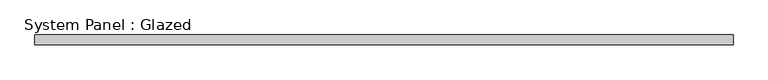
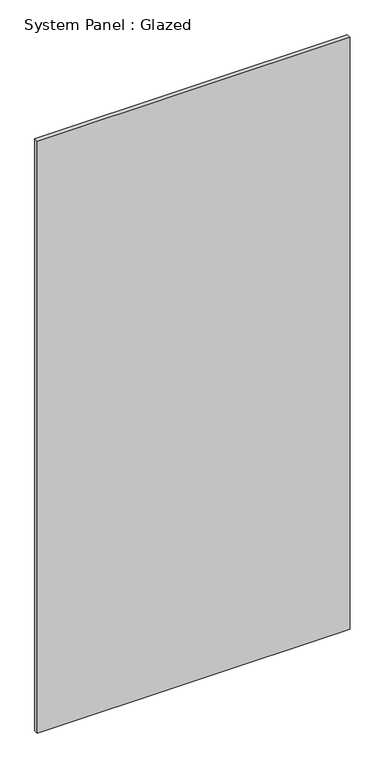
"""IFC4 building model written with IfcOpenShell, lengths in millimetres: plate geometry, System Panel : Glazed."""

import ifcopenshell
import ifcopenshell.guid

model = None  # the IFC model being written
_history = None  # IfcOwnerHistory: only IFC2X3 demands one
_inside = {}  # id of a spatial element -> (the spatial element, [elements in it])
_under = {}  # id of a project, library or spatial element -> (it, [spatial elements below it])
_declared = {}  # id of a project -> (the project, [libraries it declares])
_typed = {}  # id of a type object -> (the type object, [elements of that type])
_made_of = {}  # id of a material, layer set ... -> (it, [elements and type objects made of it])


def new_model(schema):
    """Start an empty IFC model of exactly this schema.

    Asked for "IFC4X3", IfcOpenShell would pick the latest addendum, in which some entities
    have other attributes; the version numbers below select the first issue.
    IFC2X3 requires an IfcOwnerHistory on every rooted entity: one is made here for all.
    """
    global model, _history
    if schema == "IFC4X3":
        model = ifcopenshell.file(schema_version=(4, 3, 0, 0))
    else:
        model = ifcopenshell.file(schema=schema)
    _inside.clear()
    _under.clear()
    _declared.clear()
    _typed.clear()
    _made_of.clear()
    _history = None
    if model.schema == "IFC2X3":
        org = make("IfcOrganization", Name="unknown")
        user = make(
            "IfcPersonAndOrganization",
            ThePerson=make("IfcPerson", FamilyName="unknown"),
            TheOrganization=org,
        )
        app = make(
            "IfcApplication",
            ApplicationDeveloper=org,
            Version="unknown",
            ApplicationFullName="unknown",
            ApplicationIdentifier="unknown",
        )
        _history = make(
            "IfcOwnerHistory",
            OwningUser=user,
            OwningApplication=app,
            ChangeAction="ADDED",
            CreationDate=0,
        )
    return model


def make(cls, **values):
    """One entity of the class cls with the attributes given. An attribute that is None is left unset."""
    return model.create_entity(
        cls, **{name: value for name, value in values.items() if value is not None}
    )


def rooted(cls, **values):
    """An entity with a GlobalId (a new one), such as an element, a storey or a relation."""
    return make(cls, GlobalId=ifcopenshell.guid.new(), OwnerHistory=_history, **values)


def si_unit(unit_type, name, prefix=None):
    """IfcSIUnit, for example si_unit("LENGTHUNIT", "METRE", prefix="MILLI")."""
    return make("IfcSIUnit", UnitType=unit_type, Prefix=prefix, Name=name)


def assignment(units):
    """IfcUnitAssignment: the units of a project."""
    return None if units is None else make("IfcUnitAssignment", Units=units)


def point(xyz):
    """IfcCartesianPoint."""
    return None if xyz is None else make("IfcCartesianPoint", Coordinates=xyz)


def direction(xyz):
    """IfcDirection."""
    return None if xyz is None else make("IfcDirection", DirectionRatios=xyz)


def frame(location, z_axis=None, x_axis=None):
    """IfcAxis2Placement3D, a coordinate frame: its origin and axes. An axis left out is left unset."""
    return make(
        "IfcAxis2Placement3D",
        Location=point(location),
        Axis=direction(z_axis),
        RefDirection=direction(x_axis),
    )


def origin():
    """The frame at (0, 0, 0) with its axes left unset."""
    return frame((0.0, 0.0, 0.0))


def origin_with_axes():
    """The frame at (0, 0, 0) with the z axis (0, 0, 1) and the x axis (1, 0, 0) written out."""
    return frame((0.0, 0.0, 0.0), z_axis=(0.0, 0.0, 1.0), x_axis=(1.0, 0.0, 0.0))


def place(relative_to, where):
    """IfcLocalPlacement: puts the frame where relative to a parent placement (None: the world)."""
    return make(
        "IfcLocalPlacement", PlacementRelTo=relative_to, RelativePlacement=where
    )


def context(
    kind, dimensions, precision=None, world=None, true_north=None, identifier=None
):
    """IfcGeometricRepresentationContext, for example the 3D "Model" context."""
    return make(
        "IfcGeometricRepresentationContext",
        ContextIdentifier=identifier,
        ContextType=kind,
        CoordinateSpaceDimension=dimensions,
        Precision=precision,
        WorldCoordinateSystem=world,
        TrueNorth=true_north,
    )


def project(units=None, contexts=None):
    """IfcProject with its units and contexts."""
    return rooted(
        "IfcProject",
        Name="project",
        RepresentationContexts=contexts,
        UnitsInContext=assignment(units),
    )


def spatial(cls, under=None, at=None, **own):
    """A site, building, storey or space (cls), placed at a placement, below another one or the project."""
    s = rooted(cls, ObjectPlacement=at, **own)
    if under is not None:
        _under.setdefault(under.id(), (under, []))[1].append(s)
    return s


def polyline(points):
    """IfcPolyline through the points."""
    return make("IfcPolyline", Points=[point(p) for p in points])


def outline(outer, holes=None, kind="AREA"):
    """IfcArbitraryClosedProfileDef: a profile drawn as a closed curve; with holes, ...WithVoids."""
    if holes is None:
        return make("IfcArbitraryClosedProfileDef", ProfileType=kind, OuterCurve=outer)
    return make(
        "IfcArbitraryProfileDefWithVoids",
        ProfileType=kind,
        OuterCurve=outer,
        InnerCurves=holes,
    )


def extrude(swept, where, along, depth):
    """IfcExtrudedAreaSolid: the profile swept, set in the frame where, extruded along a direction by depth."""
    return make(
        "IfcExtrudedAreaSolid",
        SweptArea=swept,
        Position=where,
        ExtrudedDirection=direction(along),
        Depth=depth,
    )


def shape(context_of_items, identifier, shape_type, items):
    """IfcShapeRepresentation: the items that make up one representation, for example the "Body"."""
    return make(
        "IfcShapeRepresentation",
        ContextOfItems=context_of_items,
        RepresentationIdentifier=identifier,
        RepresentationType=shape_type,
        Items=items,
    )


def source(mapping_origin, context_of_items, identifier, shape_type, items):
    """IfcRepresentationMap: a shape defined once, which mapped items show again and again."""
    return make(
        "IfcRepresentationMap",
        MappingOrigin=mapping_origin,
        MappedRepresentation=shape(context_of_items, identifier, shape_type, items),
    )


def transform(
    local_origin,
    x_axis=None,
    y_axis=None,
    z_axis=None,
    scale=None,
    scale2=None,
    scale3=None,
    uniform=True,
):
    """IfcCartesianTransformationOperator3D, or its non-uniform kind. x_axis, y_axis, z_axis: its Axis1, 2, 3."""
    if uniform:
        return make(
            "IfcCartesianTransformationOperator3D",
            Axis1=direction(x_axis),
            Axis2=direction(y_axis),
            LocalOrigin=point(local_origin),
            Scale=scale,
            Axis3=direction(z_axis),
        )
    return make(
        "IfcCartesianTransformationOperator3DnonUniform",
        Axis1=direction(x_axis),
        Axis2=direction(y_axis),
        LocalOrigin=point(local_origin),
        Scale=scale,
        Axis3=direction(z_axis),
        Scale2=scale2,
        Scale3=scale3,
    )


def mapped(mapping_source, mapping_target):
    """IfcMappedItem: shows the shape of a source again, moved by a transform."""
    return make(
        "IfcMappedItem", MappingSource=mapping_source, MappingTarget=mapping_target
    )


def made_of(thing, what):
    """Note that an element or type object is made of a material, layer set ...; save() writes the relation."""
    if what is not None:
        _made_of.setdefault(what.id(), (what, []))[1].append(thing)
    return thing


def element(
    cls,
    number,
    at=None,
    inside=None,
    cuts=None,
    type_object=None,
    material=None,
    context=None,
    identifier="Body",
    shape_type=None,
    held_by="IfcProductDefinitionShape",
    body=None,
    shapes=None,
    **own,
):
    """One element of the class cls, such as IfcWall. Its Tag is "e" and its number.

    at: its placement. inside: the storey or other place that contains it. cuts: it is an
    opening in that element (IfcRelVoidsElement). A single representation is given by context,
    identifier, shape_type and body (its items); several are given by shapes. held_by: the class
    of the entity that holds the representations. save() writes the other relations.
    """
    e = rooted(cls, Tag="e%d" % number, ObjectPlacement=at, **own)
    if body is not None:
        shapes = [shape(context, identifier, shape_type, body)]
    if shapes is not None:
        e.Representation = make(held_by, Representations=shapes)
    if inside is not None:
        _inside.setdefault(inside.id(), (inside, []))[1].append(e)
    if cuts is not None:
        rooted(
            "IfcRelVoidsElement", RelatingBuildingElement=cuts, RelatedOpeningElement=e
        )
    if type_object is not None:
        _typed.setdefault(type_object.id(), (type_object, []))[1].append(e)
    return made_of(e, material)


def aggregate(whole, parts):
    """IfcRelAggregates: a whole, such as a stair, and the parts it consists of."""
    return rooted("IfcRelAggregates", RelatingObject=whole, RelatedObjects=parts)


def save(model, path):
    """Write the relations noted so far, then the file.

    IfcRelAggregates (storeys below a building ...), IfcRelContainedInSpatialStructure (elements
    in a storey), IfcRelDefinesByType, IfcRelAssociatesMaterial and IfcRelDeclares: one each for
    every whole, place, type object, material and project.
    """
    for whole, parts in _under.values():
        aggregate(whole, parts)
    for where, things in _inside.values():
        rooted(
            "IfcRelContainedInSpatialStructure",
            RelatedElements=things,
            RelatingStructure=where,
        )
    for kind, things in _typed.values():
        rooted("IfcRelDefinesByType", RelatedObjects=things, RelatingType=kind)
    for what, things in _made_of.values():
        rooted("IfcRelAssociatesMaterial", RelatedObjects=things, RelatingMaterial=what)
    for by, libraries in _declared.values():
        rooted("IfcRelDeclares", RelatingContext=by, RelatedDefinitions=libraries)
    model.write(path)


def system_panel_glazed_1f34555f(model_context):
    return source(origin(), model_context, "Body", "SweptSolid", [
        extrude(outline(polyline([(914.4, -44.45), (-914.4, -44.45), (-914.4, -19.05), (914.4, -19.05), (914.4, -44.45)])), origin_with_axes(), (0.0, 0.0, 1.0), 3657.6),
    ])


if __name__ == "__main__":
    model = new_model("IFC4")
    model_context = context("Model", 3, world=origin())
    ifc_project = project(units=[si_unit("LENGTHUNIT", "METRE", prefix="MILLI")], contexts=[model_context])
    site = spatial("IfcSite", under=ifc_project)
    building = spatial("IfcBuilding", under=site)
    placement = place(None, origin())
    system_panel_glazed_shape = system_panel_glazed_1f34555f(model_context)
    element("IfcPlate", 1, ObjectType="System Panel : Glazed", at=placement, inside=building, context=model_context, shape_type="MappedRepresentation", body=[
        mapped(system_panel_glazed_shape, transform((0.0, 0.0, 0.0), x_axis=(1.0, 0.0, 0.0), y_axis=(0.0, 1.0, 0.0), z_axis=(0.0, 0.0, 1.0))),
    ])
    save(model, "model.ifc")

# Revit data of these elements
# Type "System Panel : Glazed"
#   Construction Type Id = "GSP4R"
#   Analytic Construction = "1/8 in Pilkington single glazing"
#   Visual Light Transmittance = 0.9
#   Solar Heat Gain Coefficient = 0.86
#   Heat Transfer Coefficient (U) = 1.18115 BTU/(h·ft²·°F)
#   Define Thermal Properties by = 1
# Element 1 (IfcPlate, "System Panel : Glazed")
#   Materials on its faces: "Glass"
# Materials
#   "Glass": class "Glass", colour RGB 0 128 192, transparency 0.75, Description = "Soda Lime Glass", Cost = 0
